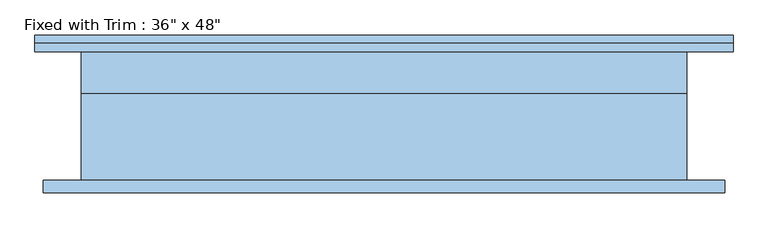
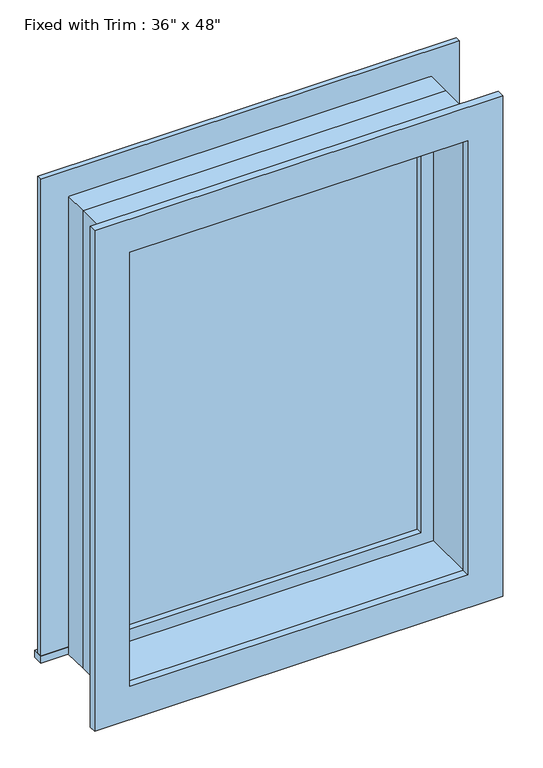
"""IFC4 building model written with IfcOpenShell, lengths in millimetres: window geometry."""

import ifcopenshell
import ifcopenshell.guid

model = None  # the IFC model being written
_history = None  # IfcOwnerHistory: only IFC2X3 demands one
_inside = {}  # id of a spatial element -> (the spatial element, [elements in it])
_under = {}  # id of a project, library or spatial element -> (it, [spatial elements below it])
_declared = {}  # id of a project -> (the project, [libraries it declares])
_typed = {}  # id of a type object -> (the type object, [elements of that type])
_made_of = {}  # id of a material, layer set ... -> (it, [elements and type objects made of it])


def new_model(schema):
    """Start an empty IFC model of exactly this schema.

    Asked for "IFC4X3", IfcOpenShell would pick the latest addendum, in which some entities
    have other attributes; the version numbers below select the first issue.
    IFC2X3 requires an IfcOwnerHistory on every rooted entity: one is made here for all.
    """
    global model, _history
    if schema == "IFC4X3":
        model = ifcopenshell.file(schema_version=(4, 3, 0, 0))
    else:
        model = ifcopenshell.file(schema=schema)
    _inside.clear()
    _under.clear()
    _declared.clear()
    _typed.clear()
    _made_of.clear()
    _history = None
    if model.schema == "IFC2X3":
        org = make("IfcOrganization", Name="unknown")
        user = make(
            "IfcPersonAndOrganization",
            ThePerson=make("IfcPerson", FamilyName="unknown"),
            TheOrganization=org,
        )
        app = make(
            "IfcApplication",
            ApplicationDeveloper=org,
            Version="unknown",
            ApplicationFullName="unknown",
            ApplicationIdentifier="unknown",
        )
        _history = make(
            "IfcOwnerHistory",
            OwningUser=user,
            OwningApplication=app,
            ChangeAction="ADDED",
            CreationDate=0,
        )
    return model


def make(cls, **values):
    """One entity of the class cls with the attributes given. An attribute that is None is left unset."""
    return model.create_entity(
        cls, **{name: value for name, value in values.items() if value is not None}
    )


def rooted(cls, **values):
    """An entity with a GlobalId (a new one), such as an element, a storey or a relation."""
    return make(cls, GlobalId=ifcopenshell.guid.new(), OwnerHistory=_history, **values)


def si_unit(unit_type, name, prefix=None):
    """IfcSIUnit, for example si_unit("LENGTHUNIT", "METRE", prefix="MILLI")."""
    return make("IfcSIUnit", UnitType=unit_type, Prefix=prefix, Name=name)


def assignment(units):
    """IfcUnitAssignment: the units of a project."""
    return None if units is None else make("IfcUnitAssignment", Units=units)


def point(xyz):
    """IfcCartesianPoint."""
    return None if xyz is None else make("IfcCartesianPoint", Coordinates=xyz)


def direction(xyz):
    """IfcDirection."""
    return None if xyz is None else make("IfcDirection", DirectionRatios=xyz)


def frame(location, z_axis=None, x_axis=None):
    """IfcAxis2Placement3D, a coordinate frame: its origin and axes. An axis left out is left unset."""
    return make(
        "IfcAxis2Placement3D",
        Location=point(location),
        Axis=direction(z_axis),
        RefDirection=direction(x_axis),
    )


def origin():
    """The frame at (0, 0, 0) with its axes left unset."""
    return frame((0.0, 0.0, 0.0))


def place(relative_to, where):
    """IfcLocalPlacement: puts the frame where relative to a parent placement (None: the world)."""
    return make(
        "IfcLocalPlacement", PlacementRelTo=relative_to, RelativePlacement=where
    )


def context(
    kind, dimensions, precision=None, world=None, true_north=None, identifier=None
):
    """IfcGeometricRepresentationContext, for example the 3D "Model" context."""
    return make(
        "IfcGeometricRepresentationContext",
        ContextIdentifier=identifier,
        ContextType=kind,
        CoordinateSpaceDimension=dimensions,
        Precision=precision,
        WorldCoordinateSystem=world,
        TrueNorth=true_north,
    )


def project(units=None, contexts=None):
    """IfcProject with its units and contexts."""
    return rooted(
        "IfcProject",
        Name="project",
        RepresentationContexts=contexts,
        UnitsInContext=assignment(units),
    )


def spatial(cls, under=None, at=None, **own):
    """A site, building, storey or space (cls), placed at a placement, below another one or the project."""
    s = rooted(cls, ObjectPlacement=at, **own)
    if under is not None:
        _under.setdefault(under.id(), (under, []))[1].append(s)
    return s


def polyline(points):
    """IfcPolyline through the points."""
    return make("IfcPolyline", Points=[point(p) for p in points])


def outline(outer, holes=None, kind="AREA"):
    """IfcArbitraryClosedProfileDef: a profile drawn as a closed curve; with holes, ...WithVoids."""
    if holes is None:
        return make("IfcArbitraryClosedProfileDef", ProfileType=kind, OuterCurve=outer)
    return make(
        "IfcArbitraryProfileDefWithVoids",
        ProfileType=kind,
        OuterCurve=outer,
        InnerCurves=holes,
    )


def extrude(swept, where, along, depth):
    """IfcExtrudedAreaSolid: the profile swept, set in the frame where, extruded along a direction by depth."""
    return make(
        "IfcExtrudedAreaSolid",
        SweptArea=swept,
        Position=where,
        ExtrudedDirection=direction(along),
        Depth=depth,
    )


def shape(context_of_items, identifier, shape_type, items):
    """IfcShapeRepresentation: the items that make up one representation, for example the "Body"."""
    return make(
        "IfcShapeRepresentation",
        ContextOfItems=context_of_items,
        RepresentationIdentifier=identifier,
        RepresentationType=shape_type,
        Items=items,
    )


def source(mapping_origin, context_of_items, identifier, shape_type, items):
    """IfcRepresentationMap: a shape defined once, which mapped items show again and again."""
    return make(
        "IfcRepresentationMap",
        MappingOrigin=mapping_origin,
        MappedRepresentation=shape(context_of_items, identifier, shape_type, items),
    )


def transform(
    local_origin,
    x_axis=None,
    y_axis=None,
    z_axis=None,
    scale=None,
    scale2=None,
    scale3=None,
    uniform=True,
):
    """IfcCartesianTransformationOperator3D, or its non-uniform kind. x_axis, y_axis, z_axis: its Axis1, 2, 3."""
    if uniform:
        return make(
            "IfcCartesianTransformationOperator3D",
            Axis1=direction(x_axis),
            Axis2=direction(y_axis),
            LocalOrigin=point(local_origin),
            Scale=scale,
            Axis3=direction(z_axis),
        )
    return make(
        "IfcCartesianTransformationOperator3DnonUniform",
        Axis1=direction(x_axis),
        Axis2=direction(y_axis),
        LocalOrigin=point(local_origin),
        Scale=scale,
        Axis3=direction(z_axis),
        Scale2=scale2,
        Scale3=scale3,
    )


def mapped(mapping_source, mapping_target):
    """IfcMappedItem: shows the shape of a source again, moved by a transform."""
    return make(
        "IfcMappedItem", MappingSource=mapping_source, MappingTarget=mapping_target
    )


def made_of(thing, what):
    """Note that an element or type object is made of a material, layer set ...; save() writes the relation."""
    if what is not None:
        _made_of.setdefault(what.id(), (what, []))[1].append(thing)
    return thing


def element(
    cls,
    number,
    at=None,
    inside=None,
    cuts=None,
    type_object=None,
    material=None,
    context=None,
    identifier="Body",
    shape_type=None,
    held_by="IfcProductDefinitionShape",
    body=None,
    shapes=None,
    **own,
):
    """One element of the class cls, such as IfcWall. Its Tag is "e" and its number.

    at: its placement. inside: the storey or other place that contains it. cuts: it is an
    opening in that element (IfcRelVoidsElement). A single representation is given by context,
    identifier, shape_type and body (its items); several are given by shapes. held_by: the class
    of the entity that holds the representations. save() writes the other relations.
    """
    e = rooted(cls, Tag="e%d" % number, ObjectPlacement=at, **own)
    if body is not None:
        shapes = [shape(context, identifier, shape_type, body)]
    if shapes is not None:
        e.Representation = make(held_by, Representations=shapes)
    if inside is not None:
        _inside.setdefault(inside.id(), (inside, []))[1].append(e)
    if cuts is not None:
        rooted(
            "IfcRelVoidsElement", RelatingBuildingElement=cuts, RelatedOpeningElement=e
        )
    if type_object is not None:
        _typed.setdefault(type_object.id(), (type_object, []))[1].append(e)
    return made_of(e, material)


def aggregate(whole, parts):
    """IfcRelAggregates: a whole, such as a stair, and the parts it consists of."""
    return rooted("IfcRelAggregates", RelatingObject=whole, RelatedObjects=parts)


def save(model, path):
    """Write the relations noted so far, then the file.

    IfcRelAggregates (storeys below a building ...), IfcRelContainedInSpatialStructure (elements
    in a storey), IfcRelDefinesByType, IfcRelAssociatesMaterial and IfcRelDeclares: one each for
    every whole, place, type object, material and project.
    """
    for whole, parts in _under.values():
        aggregate(whole, parts)
    for where, things in _inside.values():
        rooted(
            "IfcRelContainedInSpatialStructure",
            RelatedElements=things,
            RelatingStructure=where,
        )
    for kind, things in _typed.values():
        rooted("IfcRelDefinesByType", RelatedObjects=things, RelatingType=kind)
    for what, things in _made_of.values():
        rooted("IfcRelAssociatesMaterial", RelatedObjects=things, RelatingMaterial=what)
    for by, libraries in _declared.values():
        rooted("IfcRelDeclares", RelatingContext=by, RelatedDefinitions=libraries)
    model.write(path)


def window_31be35ed(model_context):
    return source(origin(), model_context, "Body", "SweptSolid", [
        extrude(outline(polyline([(-565.15, 122.2375), (488.95, 122.2375), (488.95, 96.8375), (-565.15, 96.8375), (-565.15, 122.2375)])), frame((0.0, 0.0, 914.4), z_axis=(0.0, 0.0, 1.0), x_axis=(1.0, 0.0, 0.0)), (0.0, 0.0, 1.0), 19.05),
        extrude(outline(polyline([(2114.55, -476.25), (2114.55, 400.05), (933.45, 400.05), (933.45, 488.95), (2203.45, 488.95), (2203.45, -565.15), (933.45, -565.15), (933.45, -476.25), (2114.55, -476.25)])), frame((0.0, 96.8375, 0.0), z_axis=(0.0, 1.0, 0.0), x_axis=(0.0, 0.0, 1.0)), (0.0, 0.0, 1.0), 12.7),
        extrude(outline(polyline([(2190.75, 476.25), (2190.75, -552.45), (857.25, -552.45), (857.25, 476.25), (2190.75, 476.25)]), holes=[polyline([(2101.85, 387.35), (946.15, 387.35), (946.15, -463.55), (2101.85, -463.55), (2101.85, 387.35)])]), frame((0.0, -115.8875, 0.0), z_axis=(0.0, 1.0, 0.0), x_axis=(0.0, 0.0, 1.0)), (0.0, 0.0, 1.0), 19.05),
        extrude(outline(polyline([(355.6, 49.2125), (-431.8, 49.2125), (-431.8, 61.9125), (355.6, 61.9125), (355.6, 49.2125)])), frame((0.0, 0.0, 977.9), z_axis=(0.0, 0.0, 1.0), x_axis=(1.0, 0.0, 0.0)), (0.0, 0.0, 1.0), 1092.2),
        extrude(outline(polyline([(2114.55, -476.25), (933.45, -476.25), (933.45, 400.05), (2114.55, 400.05), (2114.55, -476.25)]), holes=[polyline([(2070.1, -431.8), (2070.1, 355.6), (977.9, 355.6), (977.9, -431.8), (2070.1, -431.8)])]), frame((0.0, 33.3375, 0.0), z_axis=(0.0, 1.0, 0.0), x_axis=(0.0, 0.0, 1.0)), (0.0, 0.0, 1.0), 44.45),
        extrude(outline(polyline([(2133.6, -495.3), (914.4, -495.3), (914.4, 419.1), (2133.6, 419.1), (2133.6, -495.3)]), holes=[polyline([(2101.85, -463.55), (2101.85, 387.35), (946.15, 387.35), (946.15, -463.55), (2101.85, -463.55)])]), frame((0.0, -96.8375, 0.0), z_axis=(0.0, 1.0, 0.0), x_axis=(0.0, 0.0, 1.0)), (0.0, 0.0, 1.0), 130.175),
        extrude(outline(polyline([(2133.6, 419.1), (2133.6, -495.3), (914.4, -495.3), (914.4, 419.1), (2133.6, 419.1)]), holes=[polyline([(2114.55, 400.05), (933.45, 400.05), (933.45, -476.25), (2114.55, -476.25), (2114.55, 400.05)])]), frame((0.0, 33.3375, 0.0), z_axis=(0.0, 1.0, 0.0), x_axis=(0.0, 0.0, 1.0)), (0.0, 0.0, 1.0), 63.5),
    ])


if __name__ == "__main__":
    model = new_model("IFC4")
    model_context = context("Model", 3, world=origin())
    ifc_project = project(units=[si_unit("LENGTHUNIT", "METRE", prefix="MILLI")], contexts=[model_context])
    site = spatial("IfcSite", under=ifc_project)
    building = spatial("IfcBuilding", under=site)
    placement = place(None, origin())
    window_shape = window_31be35ed(model_context)
    element("IfcWindow", 1, ObjectType="Fixed with Trim : 36\" x 48\"", at=placement, inside=building, context=model_context, shape_type="MappedRepresentation", body=[
        mapped(window_shape, transform((0.0, 0.0, 0.0), x_axis=(1.0, 0.0, 0.0), y_axis=(0.0, 1.0, 0.0), z_axis=(0.0, 0.0, 1.0))),
    ])
    save(model, "model.ifc")

# Revit data of these elements
# Type "Fixed with Trim : 36\" x 48\""
#   Type Mark = "46"
#   Assembly Code = "B2020100"
#   Height = 4' - 0"
#   Default Sill Height = 3' - 0"
#   Trim Projection - Ext. = 0' - 0 1/2"
#   Trim Projection - Int. = 0' - 0 3/4"
#   Trim Width - Exterior = 0' - 3 1/2"
#   Trim Width - Interior = 0' - 3 1/2"
#   Width = 3' - 0"
#   Window Inset = 0' - 0 3/4"
#   Define Thermal Properties by = 0
#   Glass Pane Material = Glass
#   Sash Material = Sash
#   Trim Exterior Material = Trim
#   Trim Interior Material = Trim
#   Wall Closure = (empty or 0)
# Element 1 (IfcWindow, "Fixed with Trim : 36\" x 48\"")
#   Materials on its faces: "Sash", "Trim", "Glass"
# Materials
#   "Glass": class "Glass", colour RGB 236 240 239, transparency 0.5, Description = "Soda Lime Glass", Cost = 0
#   "Sash": class "Wood", colour RGB 227 170 128, transparency 0, Cost = 0
#   "Trim": class "Wood", colour RGB 227 170 128, transparency 0, Cost = 0
